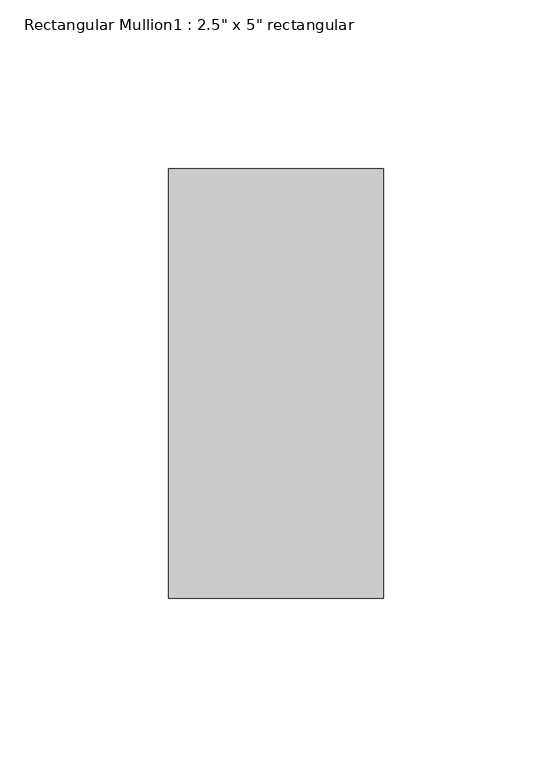
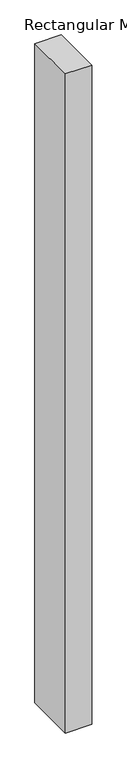
"""IFC4 building model written with IfcOpenShell, lengths in millimetres: member geometry."""

from ifc_helpers import new_model, si_unit, frame, origin, place, context, project, spatial, polyline, outline, extrude, source, transform, mapped, element, save


def member_38e9bff8(model_context):
    return source(origin(), model_context, "Body", "SweptSolid", [
        extrude(outline(polyline([(31.75, 63.5), (31.75, -63.5), (-31.75, -63.5), (-31.75, 63.5), (31.75, 63.5)])), frame((0.0, 0.0, -1676.4), z_axis=(0.0, 0.0, 1.0), x_axis=(1.0, 0.0, 0.0)), (0.0, 0.0, 1.0), 1676.4),
    ])


if __name__ == "__main__":
    model = new_model("IFC4")
    model_context = context("Model", 3, world=origin())
    ifc_project = project(units=[si_unit("LENGTHUNIT", "METRE", prefix="MILLI")], contexts=[model_context])
    site = spatial("IfcSite", under=ifc_project)
    building = spatial("IfcBuilding", under=site)
    placement = place(None, origin())
    member_shape = member_38e9bff8(model_context)
    element("IfcMember", 1, ObjectType="Rectangular Mullion1 : 2.5\" x 5\" rectangular", at=placement, inside=building, context=model_context, shape_type="MappedRepresentation", body=[
        mapped(member_shape, transform((0.0, 0.0, 0.0), x_axis=(1.0, 0.0, 0.0), y_axis=(0.0, 1.0, 0.0), z_axis=(0.0, 0.0, 1.0))),
    ])
    save(model, "model.ifc")

# Revit data of these elements
# Type "Rectangular Mullion1 : 2.5\" x 5\" rectangular"
#   built-in parameter 1007304 = 0.416667 (stored number, unit not read)
#   built-in parameter 1007301 = 0.104167 (stored number, unit not read)
#   built-in parameter 1007300 = 0.104167 (stored number, unit not read)
# Element 1 (IfcMember, "Rectangular Mullion1 : 2.5\" x 5\" rectangular")
#   Materials on its faces: "support-frame"
# Materials
#   "support-frame": class "Unassigned", colour RGB 233 233 233, transparency 0, Cost = 0
